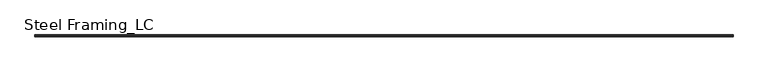
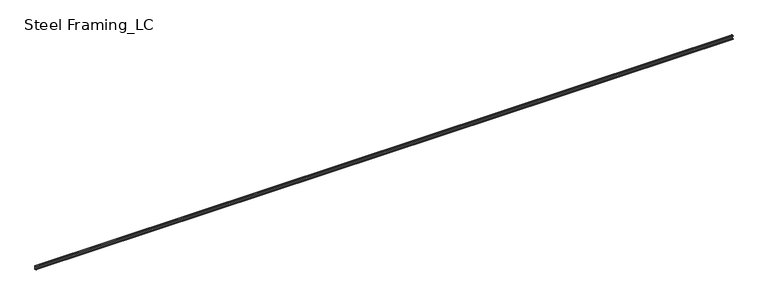
"""IFC4 building model written with IfcOpenShell, lengths in millimetres: beam geometry, Steel Framing_LC : H_SB_AR_S00_LC-150x75x25x3.2."""

from ifc_helpers import new_model, si_unit, point, frame, frame_2d, origin, place, context, project, spatial, polyline, circle_curve, trimmed, segment, composite_curve, outline, extrude, source, transform, mapped, element, save


def steel_framing_lc_7a68255c(model_context):
    return source(origin(), model_context, "Body", "SweptSolid", [
        extrude(outline(composite_curve([segment(polyline([(18.6, 67.0), (18.6, -67.0)]), True, "CONTINUOUS"), segment(trimmed(circle_curve(frame_2d((10.6, -67.0)), 8.0), [point((18.6, -67.0))], [point((10.6, -75.0))], False, "CARTESIAN"), True, "CONTINUOUS"), segment(polyline([(10.6, -75.0), (-48.4, -75.0)]), True, "CONTINUOUS"), segment(trimmed(circle_curve(frame_2d((-48.4, -67.0)), 8.0), [point((-48.4, -75.0))], [point((-56.4, -67.0))], False, "CARTESIAN"), True, "CONTINUOUS"), segment(polyline([(-56.4, -67.0), (-56.4, -50.0), (-53.2, -50.0), (-53.2, -67.0)]), True, "CONTINUOUS"), segment(trimmed(circle_curve(frame_2d((-48.4, -67.0)), 4.8), [point((-53.2, -67.0))], [point((-48.4, -71.8))], True, "CARTESIAN"), True, "CONTINUOUS"), segment(polyline([(-48.4, -71.8), (10.6, -71.8)]), True, "CONTINUOUS"), segment(trimmed(circle_curve(frame_2d((10.6, -67.0)), 4.8), [point((10.6, -71.8))], [point((15.4, -67.0))], True, "CARTESIAN"), True, "CONTINUOUS"), segment(polyline([(15.4, -67.0), (15.4, 67.0)]), True, "CONTINUOUS"), segment(trimmed(circle_curve(frame_2d((10.6, 67.0)), 4.8), [point((15.4, 67.0))], [point((10.6, 71.8))], True, "CARTESIAN"), True, "CONTINUOUS"), segment(polyline([(10.6, 71.8), (-48.4, 71.8)]), True, "CONTINUOUS"), segment(trimmed(circle_curve(frame_2d((-48.4, 67.0)), 4.8), [point((-48.4, 71.8))], [point((-53.2, 67.0))], True, "CARTESIAN"), True, "CONTINUOUS"), segment(polyline([(-53.2, 67.0), (-53.2, 50.0), (-56.4, 50.0), (-56.4, 67.0)]), True, "CONTINUOUS"), segment(trimmed(circle_curve(frame_2d((-48.4, 67.0)), 8.0), [point((-56.4, 67.0))], [point((-48.4, 75.0))], False, "CARTESIAN"), True, "CONTINUOUS"), segment(polyline([(-48.4, 75.0), (10.6, 75.0)]), True, "CONTINUOUS"), segment(trimmed(circle_curve(frame_2d((10.6, 67.0)), 8.0), [point((10.6, 75.0))], [point((18.6, 67.0))], False, "CARTESIAN"), True, "CONTINUOUS")], self_intersect=False)), frame((-15450.0, 0.0, 0.0), z_axis=(1.0, 0.0, 0.0), x_axis=(0.0, 1.0, 0.0)), (0.0, 0.0, 1.0), 30900.0),
    ])


if __name__ == "__main__":
    model = new_model("IFC4")
    model_context = context("Model", 3, world=origin())
    ifc_project = project(units=[si_unit("LENGTHUNIT", "METRE", prefix="MILLI")], contexts=[model_context])
    site = spatial("IfcSite", under=ifc_project)
    building = spatial("IfcBuilding", under=site)
    placement = place(None, origin())
    steel_framing_lc_shape = steel_framing_lc_7a68255c(model_context)
    element("IfcBeam", 1, ObjectType="Steel Framing_LC : H_SB_AR_S00_LC-150x75x25x3.2", at=placement, inside=building, context=model_context, shape_type="MappedRepresentation", body=[
        mapped(steel_framing_lc_shape, transform((0.0, 0.0, 0.0), x_axis=(1.0, 0.0, 0.0), y_axis=(0.0, 1.0, 0.0), z_axis=(0.0, 0.0, 1.0))),
    ])
    save(model, "model.ifc")

# Revit data of these elements
# Type "Steel Framing_LC : H_SB_AR_S00_LC-150x75x25x3.2"
#   Type Comments = "SECONDARY"
#   Type Mark = "GIRTH"
#   H_SectionID = "LC-150x75x25x3.2"
#   r = 4.8 mm
#   d = 25 mm
#   R = 8 mm
#   Perimeter = 0.70 m²/m
#   Nominal Weight = 10.30 kgf/m
#   Length [instance default] = 1000 mm
#   b = 75 mm
#   h = 150 mm
#   tw = 3.2 mm
#   x = 18.6 mm
#   A = 1.00 m²
#   Structural Material [instance default] = Steel, 45-345
#   Assembly Code = ""
# Element 1 (IfcBeam, "Steel Framing_LC : H_SB_AR_S00_LC-150x75x25x3.2")
#   Materials on its faces: "Steel, 45-345"
# Materials
#   "Steel, 45-345": class "Metal", colour RGB 189 187 185, transparency 0, Description = "Steel 345 MPa", Cost = 0
